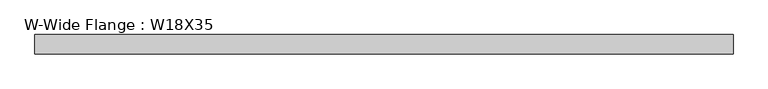
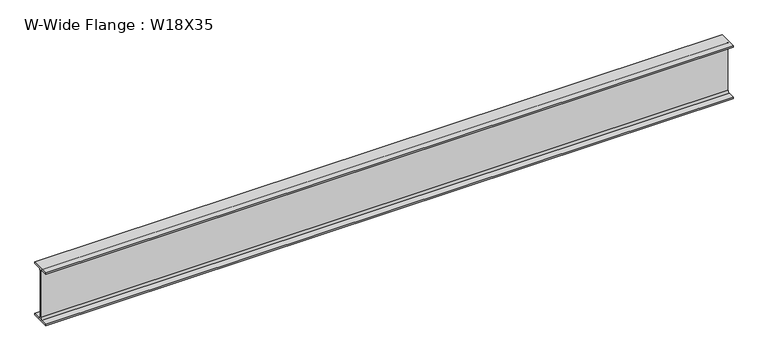
"""IFC4 building model written with IfcOpenShell, lengths in millimetres: beam geometry, W-Wide Flange : W18X35."""

from ifc_helpers import new_model, si_unit, point, frame, frame_2d, origin, place, context, project, spatial, polyline, circle_curve, trimmed, segment, composite_curve, outline, extrude, source, transform, mapped, element, save


def w_wide_flange_w18x35_c5c9a120(model_context):
    return source(origin(), model_context, "Body", "SweptSolid", [
        extrude(outline(composite_curve([segment(polyline([(76.2, -213.995), (76.2, -224.79), (-76.2, -224.79), (-76.2, -213.995), (-21.59, -213.995)]), True, "CONTINUOUS"), segment(trimmed(circle_curve(frame_2d((-21.59, -196.215)), 17.78), [point((-21.59, -213.995))], [point((-3.81, -196.215))], True, "CARTESIAN"), True, "CONTINUOUS"), segment(polyline([(-3.81, -196.215), (-3.81, 196.215)]), True, "CONTINUOUS"), segment(trimmed(circle_curve(frame_2d((-21.59, 196.215)), 17.78), [point((-3.81, 196.215))], [point((-21.59, 213.995))], True, "CARTESIAN"), True, "CONTINUOUS"), segment(polyline([(-21.59, 213.995), (-76.2, 213.995), (-76.2, 224.79), (76.2, 224.79), (76.2, 213.995), (21.59, 213.995)]), True, "CONTINUOUS"), segment(trimmed(circle_curve(frame_2d((21.59, 196.215)), 17.78), [point((21.59, 213.995))], [point((3.81, 196.215))], True, "CARTESIAN"), True, "CONTINUOUS"), segment(polyline([(3.81, 196.215), (3.81, -196.215)]), True, "CONTINUOUS"), segment(trimmed(circle_curve(frame_2d((21.59, -196.215)), 17.78), [point((3.81, -196.215))], [point((21.59, -213.995))], True, "CARTESIAN"), True, "CONTINUOUS"), segment(polyline([(21.59, -213.995), (76.2, -213.995)]), True, "CONTINUOUS")], self_intersect=False)), frame((-2755.9, 0.0, 0.0), z_axis=(1.0, 0.0, 0.0), x_axis=(0.0, 1.0, 0.0)), (0.0, 0.0, 1.0), 5539.2574),
    ])


if __name__ == "__main__":
    model = new_model("IFC4")
    model_context = context("Model", 3, world=origin())
    ifc_project = project(units=[si_unit("LENGTHUNIT", "METRE", prefix="MILLI")], contexts=[model_context])
    site = spatial("IfcSite", under=ifc_project)
    building = spatial("IfcBuilding", under=site)
    placement = place(None, origin())
    w_wide_flange_w18x35_shape = w_wide_flange_w18x35_c5c9a120(model_context)
    element("IfcBeam", 1, ObjectType="W-Wide Flange : W18X35", at=placement, inside=building, context=model_context, shape_type="MappedRepresentation", body=[
        mapped(w_wide_flange_w18x35_shape, transform((0.0, 0.0, 0.0), x_axis=(1.0, 0.0, 0.0), y_axis=(0.0, 1.0, 0.0), z_axis=(0.0, 0.0, 1.0))),
    ])
    save(model, "model.ifc")

# Revit data of these elements
# Type "W-Wide Flange : W18X35"
#   Assembly Code = "B10"
#   W = 35
#   Length [instance default] = 5' - 0"
#   bf = 0' - 6"
#   d = 1' - 5.7"
#   k = 0' - 1 1/8"
#   k2 = 0' - 0.7"
#   tf = 0' - 0.425"
#   tw = 0' - 0.3"
#   A = 0.0715278 SF
#   Structural Material [instance default] = Steel ASTM A992
# Element 1 (IfcBeam, "W-Wide Flange : W18X35")
#   Materials on its faces: "Steel ASTM A992"
# Materials
#   "Steel ASTM A992": class "Metal", colour RGB 199 199 199, transparency 0, Description = "Structural steel 50ksi", Cost = 0
